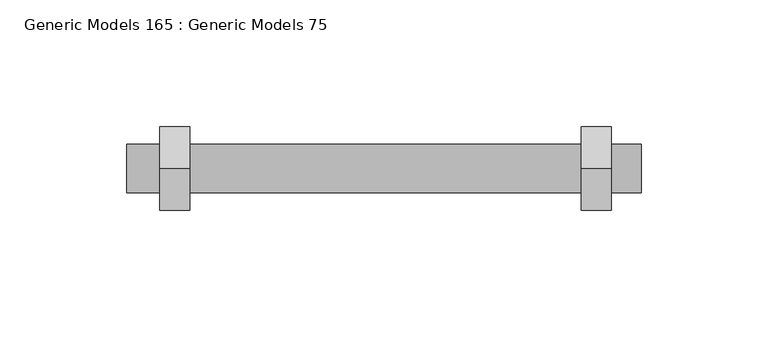
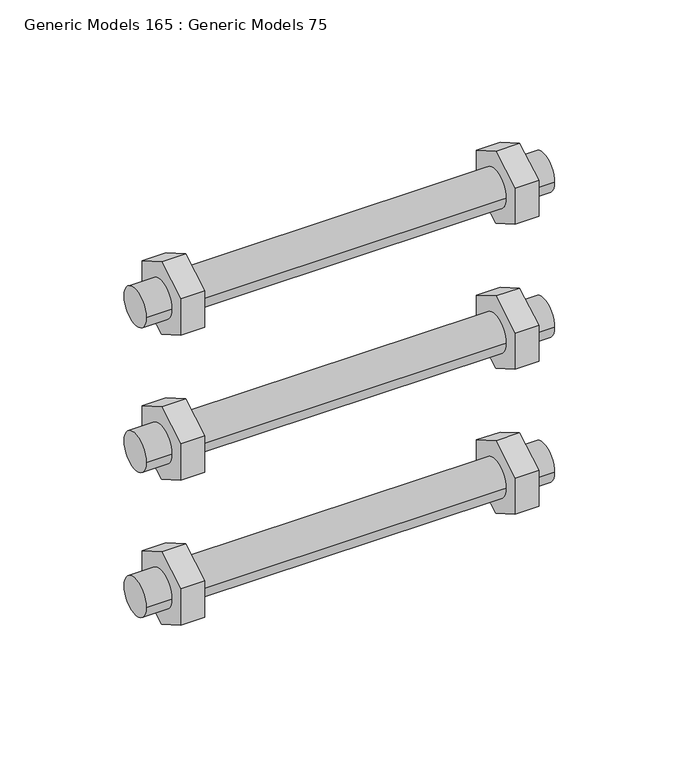
"""IFC4 building model written with IfcOpenShell, lengths in millimetres: proxy geometry, Generic Models 165 : Generic Models 75."""

from ifc_helpers import new_model, si_unit, point, frame, frame_2d, origin, place, context, project, spatial, polyline, circle_curve, trimmed, segment, composite_curve, outline, extrude, source, transform, mapped, element, save


def generic_models_165_generic_models_75_19e53021(model_context):
    return source(origin(), model_context, "Body", "SweptSolid", [
        extrude(outline(polyline([(36285.0123281, 271852.097122), (36285.0123281, 271833.047122), (36268.5145442, 271823.522122), (36252.0167603, 271833.047122), (36252.0167603, 271852.097122), (36268.5145442, 271861.622122), (36285.0123281, 271852.097122)])), frame((31918.2596032, 0.0, 0.0), z_axis=(1.0, 0.0, 0.0), x_axis=(0.0, 1.0, 0.0)), (0.0, 0.0, 1.0), 11.90625),
        extrude(outline(polyline([(36285.0123281, 271775.897122), (36285.0123281, 271756.847122), (36268.5145442, 271747.322122), (36252.0167603, 271756.847122), (36252.0167603, 271775.897122), (36268.5145442, 271785.422122), (36285.0123281, 271775.897122)])), frame((31918.2596032, 0.0, 0.0), z_axis=(1.0, 0.0, 0.0), x_axis=(0.0, 1.0, 0.0)), (0.0, 0.0, 1.0), 11.90625),
        extrude(outline(polyline([(36285.0123281, 271699.697122), (36285.0123281, 271680.647122), (36268.5145442, 271671.122122), (36252.0167603, 271680.647122), (36252.0167603, 271699.697122), (36268.5145442, 271709.222122), (36285.0123281, 271699.697122)])), frame((31918.2596032, 0.0, 0.0), z_axis=(1.0, 0.0, 0.0), x_axis=(0.0, 1.0, 0.0)), (0.0, 0.0, 1.0), 11.90625),
        extrude(outline(polyline([(36285.0123281, 271852.097122), (36285.0123281, 271833.047122), (36268.5145442, 271823.522122), (36252.0167603, 271833.047122), (36252.0167603, 271852.097122), (36268.5145442, 271861.622122), (36285.0123281, 271852.097122)])), frame((31751.9689782, 0.0, 0.0), z_axis=(1.0, 0.0, 0.0), x_axis=(0.0, 1.0, 0.0)), (0.0, 0.0, 1.0), 11.90625),
        extrude(outline(polyline([(36285.0123281, 271775.897122), (36285.0123281, 271756.847122), (36268.5145442, 271747.322122), (36252.0167603, 271756.847122), (36252.0167603, 271775.897122), (36268.5145442, 271785.422122), (36285.0123281, 271775.897122)])), frame((31751.9689782, 0.0, 0.0), z_axis=(1.0, 0.0, 0.0), x_axis=(0.0, 1.0, 0.0)), (0.0, 0.0, 1.0), 11.90625),
        extrude(outline(polyline([(36285.0123281, 271699.697122), (36285.0123281, 271680.647122), (36268.5145442, 271671.122122), (36252.0167603, 271680.647122), (36252.0167603, 271699.697122), (36268.5145442, 271709.222122), (36285.0123281, 271699.697122)])), frame((31751.9689782, 0.0, 0.0), z_axis=(1.0, 0.0, 0.0), x_axis=(0.0, 1.0, 0.0)), (0.0, 0.0, 1.0), 11.90625),
        extrude(outline(composite_curve([segment(trimmed(circle_curve(frame_2d((36268.5145442, 271766.372122)), 9.525), [point((36258.9895442, 271766.372122))], [point((36278.0395442, 271766.372122))], False, "CARTESIAN"), True, "CONTINUOUS"), segment(trimmed(circle_curve(frame_2d((36268.5145442, 271766.372122)), 9.525), [point((36278.0395442, 271766.372122))], [point((36258.9895442, 271766.372122))], False, "CARTESIAN"), True, "CONTINUOUS")], self_intersect=False)), frame((31738.8721032, 0.0, 0.0), z_axis=(1.0, 0.0, 0.0), x_axis=(0.0, 1.0, 0.0)), (0.0, 0.0, 1.0), 203.2),
        extrude(outline(composite_curve([segment(trimmed(circle_curve(frame_2d((36268.5145442, 271690.172122)), 9.525), [point((36258.9895442, 271690.172122))], [point((36278.0395442, 271690.172122))], False, "CARTESIAN"), True, "CONTINUOUS"), segment(trimmed(circle_curve(frame_2d((36268.5145442, 271690.172122)), 9.525), [point((36278.0395442, 271690.172122))], [point((36258.9895442, 271690.172122))], False, "CARTESIAN"), True, "CONTINUOUS")], self_intersect=False)), frame((31738.8721032, 0.0, 0.0), z_axis=(1.0, 0.0, 0.0), x_axis=(0.0, 1.0, 0.0)), (0.0, 0.0, 1.0), 203.2),
        extrude(outline(composite_curve([segment(trimmed(circle_curve(frame_2d((36268.5145442, 271842.572122)), 9.525), [point((36258.9895442, 271842.572122))], [point((36278.0395442, 271842.572122))], False, "CARTESIAN"), True, "CONTINUOUS"), segment(trimmed(circle_curve(frame_2d((36268.5145442, 271842.572122)), 9.525), [point((36278.0395442, 271842.572122))], [point((36258.9895442, 271842.572122))], False, "CARTESIAN"), True, "CONTINUOUS")], self_intersect=False)), frame((31738.8721032, 0.0, 0.0), z_axis=(1.0, 0.0, 0.0), x_axis=(0.0, 1.0, 0.0)), (0.0, 0.0, 1.0), 203.2),
    ])


if __name__ == "__main__":
    model = new_model("IFC4")
    model_context = context("Model", 3, world=origin())
    ifc_project = project(units=[si_unit("LENGTHUNIT", "METRE", prefix="MILLI")], contexts=[model_context])
    site = spatial("IfcSite", under=ifc_project)
    building = spatial("IfcBuilding", under=site)
    placement = place(None, origin())
    generic_models_165_generic_models_75_shape = generic_models_165_generic_models_75_19e53021(model_context)
    element("IfcBuildingElementProxy", 1, Name="Generic Models 165 : Generic Models 75", ObjectType="Generic Models 165 : Generic Models 75", at=placement, inside=building, context=model_context, shape_type="MappedRepresentation", body=[
        mapped(generic_models_165_generic_models_75_shape, transform((0.0, 0.0, 0.0), x_axis=(1.0, 0.0, 0.0), y_axis=(0.0, 1.0, 0.0), z_axis=(0.0, 0.0, 1.0))),
    ])
    save(model, "model.ifc")
